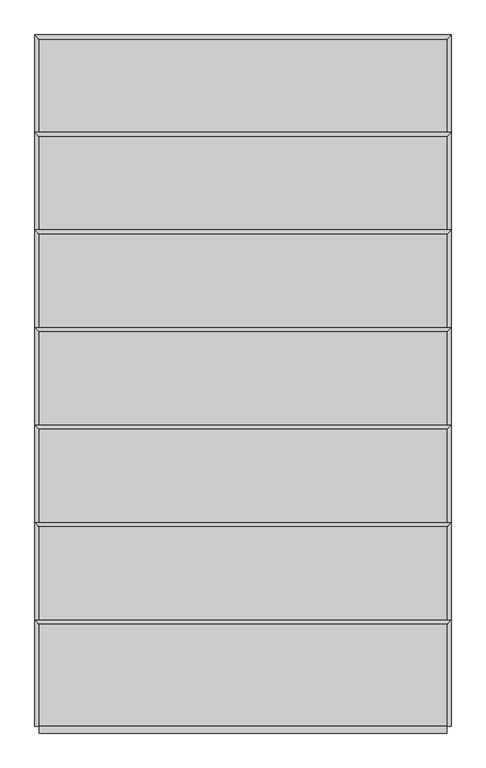
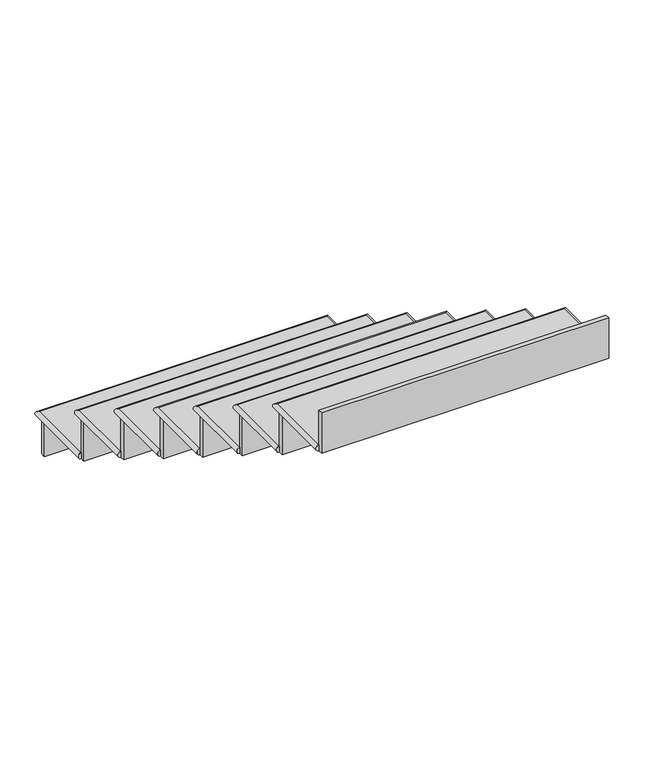
"""IFC4 building model written with IfcOpenShell, lengths in millimetres: stair flight geometry."""

import ifcopenshell
import ifcopenshell.guid

model = None  # the IFC model being written
_history = None  # IfcOwnerHistory: only IFC2X3 demands one
_inside = {}  # id of a spatial element -> (the spatial element, [elements in it])
_under = {}  # id of a project, library or spatial element -> (it, [spatial elements below it])
_declared = {}  # id of a project -> (the project, [libraries it declares])
_typed = {}  # id of a type object -> (the type object, [elements of that type])
_made_of = {}  # id of a material, layer set ... -> (it, [elements and type objects made of it])


def new_model(schema):
    """Start an empty IFC model of exactly this schema.

    Asked for "IFC4X3", IfcOpenShell would pick the latest addendum, in which some entities
    have other attributes; the version numbers below select the first issue.
    IFC2X3 requires an IfcOwnerHistory on every rooted entity: one is made here for all.
    """
    global model, _history
    if schema == "IFC4X3":
        model = ifcopenshell.file(schema_version=(4, 3, 0, 0))
    else:
        model = ifcopenshell.file(schema=schema)
    _inside.clear()
    _under.clear()
    _declared.clear()
    _typed.clear()
    _made_of.clear()
    _history = None
    if model.schema == "IFC2X3":
        org = make("IfcOrganization", Name="unknown")
        user = make(
            "IfcPersonAndOrganization",
            ThePerson=make("IfcPerson", FamilyName="unknown"),
            TheOrganization=org,
        )
        app = make(
            "IfcApplication",
            ApplicationDeveloper=org,
            Version="unknown",
            ApplicationFullName="unknown",
            ApplicationIdentifier="unknown",
        )
        _history = make(
            "IfcOwnerHistory",
            OwningUser=user,
            OwningApplication=app,
            ChangeAction="ADDED",
            CreationDate=0,
        )
    return model


def make(cls, **values):
    """One entity of the class cls with the attributes given. An attribute that is None is left unset."""
    return model.create_entity(
        cls, **{name: value for name, value in values.items() if value is not None}
    )


def rooted(cls, **values):
    """An entity with a GlobalId (a new one), such as an element, a storey or a relation."""
    return make(cls, GlobalId=ifcopenshell.guid.new(), OwnerHistory=_history, **values)


def si_unit(unit_type, name, prefix=None):
    """IfcSIUnit, for example si_unit("LENGTHUNIT", "METRE", prefix="MILLI")."""
    return make("IfcSIUnit", UnitType=unit_type, Prefix=prefix, Name=name)


def assignment(units):
    """IfcUnitAssignment: the units of a project."""
    return None if units is None else make("IfcUnitAssignment", Units=units)


def point(xyz):
    """IfcCartesianPoint."""
    return None if xyz is None else make("IfcCartesianPoint", Coordinates=xyz)


def direction(xyz):
    """IfcDirection."""
    return None if xyz is None else make("IfcDirection", DirectionRatios=xyz)


def frame(location, z_axis=None, x_axis=None):
    """IfcAxis2Placement3D, a coordinate frame: its origin and axes. An axis left out is left unset."""
    return make(
        "IfcAxis2Placement3D",
        Location=point(location),
        Axis=direction(z_axis),
        RefDirection=direction(x_axis),
    )


def origin():
    """The frame at (0, 0, 0) with its axes left unset."""
    return frame((0.0, 0.0, 0.0))


def place(relative_to, where):
    """IfcLocalPlacement: puts the frame where relative to a parent placement (None: the world)."""
    return make(
        "IfcLocalPlacement", PlacementRelTo=relative_to, RelativePlacement=where
    )


def context(
    kind, dimensions, precision=None, world=None, true_north=None, identifier=None
):
    """IfcGeometricRepresentationContext, for example the 3D "Model" context."""
    return make(
        "IfcGeometricRepresentationContext",
        ContextIdentifier=identifier,
        ContextType=kind,
        CoordinateSpaceDimension=dimensions,
        Precision=precision,
        WorldCoordinateSystem=world,
        TrueNorth=true_north,
    )


def project(units=None, contexts=None):
    """IfcProject with its units and contexts."""
    return rooted(
        "IfcProject",
        Name="project",
        RepresentationContexts=contexts,
        UnitsInContext=assignment(units),
    )


def spatial(cls, under=None, at=None, **own):
    """A site, building, storey or space (cls), placed at a placement, below another one or the project."""
    s = rooted(cls, ObjectPlacement=at, **own)
    if under is not None:
        _under.setdefault(under.id(), (under, []))[1].append(s)
    return s


def circle_curve(where, radius):
    """IfcCircle in the frame where."""
    return make("IfcCircle", Position=where, Radius=radius)


def ellipse_curve(where, semi_axis1, semi_axis2):
    """IfcEllipse in the frame where."""
    return make(
        "IfcEllipse", Position=where, SemiAxis1=semi_axis1, SemiAxis2=semi_axis2
    )


def faces_of(points, faces, orient=None, outer=None):
    """IfcFace entities. A face is a list of loops; a loop is a list of indices into points, from 0.

    orient and outer hold one flag for each loop. By default every Orientation is true, the
    first loop of a face is its IfcFaceOuterBound and the others are IfcFaceBound.
    """
    made = []
    for i, loops in enumerate(faces):
        bounds = []
        for j, loop in enumerate(loops):
            is_outer = j == 0 if outer is None else outer[i][j]
            bounds.append(
                make(
                    "IfcFaceOuterBound" if is_outer else "IfcFaceBound",
                    Bound=make("IfcPolyLoop", Polygon=[points[k] for k in loop]),
                    Orientation=True if orient is None else orient[i][j],
                )
            )
        made.append(make("IfcFace", Bounds=bounds))
    return made


def faceted_brep(points, faces, orient=None, outer=None, voids=None):
    """IfcFacetedBrep: a solid bounded by flat faces; with voids (closed shells), ...WithVoids."""
    shared = [point(p) for p in points]
    hull = make("IfcClosedShell", CfsFaces=faces_of(shared, faces, orient, outer))
    if voids is None:
        return make("IfcFacetedBrep", Outer=hull)
    return make(
        "IfcFacetedBrepWithVoids",
        Outer=hull,
        Voids=[
            make(cls, CfsFaces=faces_of(shared, fs, o, b)) for cls, fs, o, b in voids
        ],
    )


def shape(context_of_items, identifier, shape_type, items):
    """IfcShapeRepresentation: the items that make up one representation, for example the "Body"."""
    return make(
        "IfcShapeRepresentation",
        ContextOfItems=context_of_items,
        RepresentationIdentifier=identifier,
        RepresentationType=shape_type,
        Items=items,
    )


def source(mapping_origin, context_of_items, identifier, shape_type, items):
    """IfcRepresentationMap: a shape defined once, which mapped items show again and again."""
    return make(
        "IfcRepresentationMap",
        MappingOrigin=mapping_origin,
        MappedRepresentation=shape(context_of_items, identifier, shape_type, items),
    )


def transform(
    local_origin,
    x_axis=None,
    y_axis=None,
    z_axis=None,
    scale=None,
    scale2=None,
    scale3=None,
    uniform=True,
):
    """IfcCartesianTransformationOperator3D, or its non-uniform kind. x_axis, y_axis, z_axis: its Axis1, 2, 3."""
    if uniform:
        return make(
            "IfcCartesianTransformationOperator3D",
            Axis1=direction(x_axis),
            Axis2=direction(y_axis),
            LocalOrigin=point(local_origin),
            Scale=scale,
            Axis3=direction(z_axis),
        )
    return make(
        "IfcCartesianTransformationOperator3DnonUniform",
        Axis1=direction(x_axis),
        Axis2=direction(y_axis),
        LocalOrigin=point(local_origin),
        Scale=scale,
        Axis3=direction(z_axis),
        Scale2=scale2,
        Scale3=scale3,
    )


def mapped(mapping_source, mapping_target):
    """IfcMappedItem: shows the shape of a source again, moved by a transform."""
    return make(
        "IfcMappedItem", MappingSource=mapping_source, MappingTarget=mapping_target
    )


def made_of(thing, what):
    """Note that an element or type object is made of a material, layer set ...; save() writes the relation."""
    if what is not None:
        _made_of.setdefault(what.id(), (what, []))[1].append(thing)
    return thing


def element(
    cls,
    number,
    at=None,
    inside=None,
    cuts=None,
    type_object=None,
    material=None,
    context=None,
    identifier="Body",
    shape_type=None,
    held_by="IfcProductDefinitionShape",
    body=None,
    shapes=None,
    **own,
):
    """One element of the class cls, such as IfcWall. Its Tag is "e" and its number.

    at: its placement. inside: the storey or other place that contains it. cuts: it is an
    opening in that element (IfcRelVoidsElement). A single representation is given by context,
    identifier, shape_type and body (its items); several are given by shapes. held_by: the class
    of the entity that holds the representations. save() writes the other relations.
    """
    e = rooted(cls, Tag="e%d" % number, ObjectPlacement=at, **own)
    if body is not None:
        shapes = [shape(context, identifier, shape_type, body)]
    if shapes is not None:
        e.Representation = make(held_by, Representations=shapes)
    if inside is not None:
        _inside.setdefault(inside.id(), (inside, []))[1].append(e)
    if cuts is not None:
        rooted(
            "IfcRelVoidsElement", RelatingBuildingElement=cuts, RelatedOpeningElement=e
        )
    if type_object is not None:
        _typed.setdefault(type_object.id(), (type_object, []))[1].append(e)
    return made_of(e, material)


def aggregate(whole, parts):
    """IfcRelAggregates: a whole, such as a stair, and the parts it consists of."""
    return rooted("IfcRelAggregates", RelatingObject=whole, RelatedObjects=parts)


def save(model, path):
    """Write the relations noted so far, then the file.

    IfcRelAggregates (storeys below a building ...), IfcRelContainedInSpatialStructure (elements
    in a storey), IfcRelDefinesByType, IfcRelAssociatesMaterial and IfcRelDeclares: one each for
    every whole, place, type object, material and project.
    """
    for whole, parts in _under.values():
        aggregate(whole, parts)
    for where, things in _inside.values():
        rooted(
            "IfcRelContainedInSpatialStructure",
            RelatedElements=things,
            RelatingStructure=where,
        )
    for kind, things in _typed.values():
        rooted("IfcRelDefinesByType", RelatedObjects=things, RelatingType=kind)
    for what, things in _made_of.values():
        rooted("IfcRelAssociatesMaterial", RelatedObjects=things, RelatingMaterial=what)
    for by, libraries in _declared.values():
        rooted("IfcRelDeclares", RelatingContext=by, RelatedDefinitions=libraries)
    model.write(path)


def plane_surface(at):
    """IfcPlane: the flat surface through the origin of the frame at, square to its z axis."""
    return make("IfcPlane", Position=at)


def cylinder_surface(at, radius):
    """IfcCylindricalSurface: all points at the distance radius from the z axis of the frame at."""
    return make("IfcCylindricalSurface", Position=at, Radius=radius)


def advanced_brep(points, edges, surfaces, faces):
    """IfcAdvancedBrep: a solid bounded by faces that lie on surfaces and meet in shared edges.

    An edge is (start, end): straight between two places in points (the first is 0);
    or (start, end, curve); or (start, end, curve, False) where it runs against its curve.
    A face is (place in surfaces, loops), or (place, loops, False) where it looks against
    its surface's normal. A loop lists edges by number (the first is 1), with a minus sign
    where the edge is run from its end to its start. The first loop is the outer one.
    """
    corners = [point(p) for p in points]
    vertices = [make("IfcVertexPoint", VertexGeometry=c) for c in corners]
    made = []
    for start, end, *more in edges:
        made.append(
            make(
                "IfcEdgeCurve",
                EdgeStart=vertices[start],
                EdgeEnd=vertices[end],
                EdgeGeometry=more[0] if more else make("IfcPolyline", Points=[corners[start], corners[end]]),
                SameSense=more[1] if len(more) > 1 else True,
            )
        )
    hull = []
    for where, loops, *sense in faces:
        bounds = []
        for j, loop in enumerate(loops):
            ring = [make("IfcOrientedEdge", EdgeElement=made[abs(k) - 1], Orientation=k > 0) for k in loop]
            bounds.append(
                make(
                    "IfcFaceOuterBound" if j == 0 else "IfcFaceBound",
                    Bound=make("IfcEdgeLoop", EdgeList=ring),
                    Orientation=True,
                )
            )
        hull.append(make("IfcAdvancedFace", Bounds=bounds, FaceSurface=surfaces[where], SameSense=sense[0] if sense else True))
    return make("IfcAdvancedBrep", Outer=make("IfcClosedShell", CfsFaces=hull))


def stair_flight_dc9404dc(model_context):
    return source(origin(), model_context, "Body", "SolidModel", [
        advanced_brep(
        [(27220.0620052, 5811.3043237, 149.621875), (27220.0620052, 5811.3043237, 175.021875), (28388.4620052, 5811.3043237, 175.021875), (28388.4620052, 5811.3043237, 149.621875), (27220.0620052, 5519.2043237, 175.021875), (28388.4620052, 5519.2043237, 175.021875), (28388.4620052, 5519.2043237, 149.621875), (27220.0620052, 5519.2043237, 149.621875)],
        [
            (0, 1, ellipse_curve(frame((27220.0620052, 5811.3043237, 162.321875), z_axis=(0.7071067811865434, 0.7071067811865517, 0.0), x_axis=(-0.7071067811865517, 0.7071067811865434, 0.0)), 17.9605122, 12.7)),
            (1, 2),
            (2, 3, ellipse_curve(frame((28388.4620052, 5811.3043237, 162.321875), z_axis=(-0.7071067811865517, 0.7071067811865434, 0.0), x_axis=(-0.7071067811865434, -0.7071067811865516, 0.0)), 17.9605122, 12.7)),
            (3, 0),
            (4, 5),
            (5, 2),
            (1, 4),
            (6, 7),
            (7, 0),
            (3, 6),
            (4, 7, circle_curve(frame((27220.0620052, 5519.2043237, 162.321875), z_axis=(0.0, -1.0, 0.0), x_axis=(1.0, 0.0, 0.0)), 12.7)),
            (6, 5, circle_curve(frame((28388.4620052, 5519.2043237, 162.321875), z_axis=(0.0, -1.0, 0.0), x_axis=(-1.0, 0.0, 0.0)), 12.7)),
        ],
        [
            cylinder_surface(frame((27220.0620052, 5811.3043237, 162.321875), z_axis=(-1.0, 0.0, 0.0), x_axis=(0.0, -1.0, 0.0)), 12.7),
            plane_surface(frame((28388.4620052, 5824.0043237, 175.021875), z_axis=(0.0, 0.0, 1.0), x_axis=(0.0, 1.0, 0.0))),
            plane_surface(frame((28388.4620052, 5824.0043237, 149.621875), z_axis=(0.0, 0.0, -1.0), x_axis=(0.0, -1.0, 0.0))),
            plane_surface(frame((27220.0620052, 5519.2043237, 175.021875), z_axis=(0.0, -1.0, 0.0), x_axis=(0.0, 0.0, -1.0))),
            cylinder_surface(frame((27220.0620052, 5519.2043237, 162.321875), z_axis=(0.0, -1.0, 0.0), x_axis=(1.0, 0.0, 0.0)), 12.7),
            cylinder_surface(frame((28388.4620052, 5811.3043237, 162.321875), z_axis=(0.0, 1.0, 0.0), x_axis=(-1.0, 0.0, 0.0)), 12.7),
        ],
        [
            (0, [[1, 2, 3, 4]]),
            (1, [[5, 6, -2, 7]]),
            (2, [[8, 9, -4, 10]]),
            (3, [[-5, 11, -8, 12]]),
            (4, [[-11, -7, -1, -9]]),
            (5, [[-3, -6, -12, -10]]),
        ],
    ),
        faceted_brep([(27220.0620052, 5798.6043237, 149.621875), (27220.0620052, 5798.6043237, 0.0), (27220.0620052, 5779.5543237, 0.0), (27220.0620052, 5779.5543237, 149.621875), (28388.4620052, 5798.6043237, 149.621875), (28388.4620052, 5779.5543237, 149.621875), (28388.4620052, 5779.5543237, 0.0), (28388.4620052, 5798.6043237, 0.0)], [[[0, 1, 2, 3]], [[4, 5, 6, 7]], [[1, 0, 4, 7]], [[2, 1, 7, 6]], [[3, 2, 6, 5]], [[0, 3, 5, 4]]]),
        faceted_brep([(27220.0620052, 5519.2043237, 324.64375), (27220.0620052, 5519.2043237, 149.621875), (27220.0620052, 5500.1543237, 149.621875), (27220.0620052, 5500.1543237, 324.64375), (28388.4620052, 5519.2043237, 324.64375), (28388.4620052, 5500.1543237, 324.64375), (28388.4620052, 5500.1543237, 149.621875), (28388.4620052, 5519.2043237, 149.621875)], [[[0, 1, 2, 3]], [[4, 5, 6, 7]], [[1, 0, 4, 7]], [[2, 1, 7, 6]], [[3, 2, 6, 5]], [[0, 3, 5, 4]]]),
        advanced_brep(
        [(27220.0620052, 5239.8043237, 350.04375), (28388.4620052, 5239.8043237, 350.04375), (28388.4620052, 5531.9043237, 350.04375), (27220.0620052, 5531.9043237, 350.04375), (28388.4620052, 5239.8043237, 324.64375), (27220.0620052, 5239.8043237, 324.64375), (27220.0620052, 5531.9043237, 324.64375), (28388.4620052, 5531.9043237, 324.64375)],
        [
            (0, 1),
            (1, 2),
            (2, 3),
            (3, 0),
            (4, 5),
            (5, 6),
            (6, 7),
            (7, 4),
            (0, 5, circle_curve(frame((27220.0620052, 5239.8043237, 337.34375), z_axis=(0.0, -1.0, 0.0), x_axis=(1.0, 0.0, 0.0)), 12.7)),
            (4, 1, circle_curve(frame((28388.4620052, 5239.8043237, 337.34375), z_axis=(0.0, -1.0, 0.0), x_axis=(-1.0, 0.0, 0.0)), 12.7)),
            (6, 3, ellipse_curve(frame((27220.0620052, 5531.9043237, 337.34375), z_axis=(0.7071067811865378, 0.7071067811865571, 0.0), x_axis=(-0.7071067811865572, 0.7071067811865377, 0.0)), 17.9605122, 12.7)),
            (2, 7, ellipse_curve(frame((28388.4620052, 5531.9043237, 337.34375), z_axis=(-0.7071067811865572, 0.7071067811865378, 0.0), x_axis=(-0.7071067811865378, -0.7071067811865572, 0.0)), 17.9605122, 12.7)),
        ],
        [
            plane_surface(frame((28388.4620052, 5824.0043237, 350.04375), z_axis=(0.0, 0.0, 1.0), x_axis=(0.0, 1.0, 0.0))),
            plane_surface(frame((28388.4620052, 5824.0043237, 324.64375), z_axis=(0.0, 0.0, -1.0), x_axis=(0.0, -1.0, 0.0))),
            plane_surface(frame((27220.0620052, 5239.8043237, 350.04375), z_axis=(0.0, -1.0, 0.0), x_axis=(0.0, 0.0, -1.0))),
            cylinder_surface(frame((27220.0620052, 5531.9043237, 337.34375), z_axis=(-1.0, 0.0, 0.0), x_axis=(0.0, -1.0, 0.0)), 12.7),
            cylinder_surface(frame((27220.0620052, 5239.8043237, 337.34375), z_axis=(0.0, -1.0, 0.0), x_axis=(1.0, 0.0, 0.0)), 12.7),
            cylinder_surface(frame((28388.4620052, 5531.9043237, 337.34375), z_axis=(0.0, 1.0, 0.0), x_axis=(-1.0, 0.0, 0.0)), 12.7),
        ],
        [
            (0, [[1, 2, 3, 4]]),
            (1, [[5, 6, 7, 8]]),
            (2, [[-1, 9, -5, 10]]),
            (3, [[11, -3, 12, -7]]),
            (4, [[-9, -4, -11, -6]]),
            (5, [[-12, -2, -10, -8]]),
        ],
    ),
        faceted_brep([(27220.0620052, 5239.8043237, 499.665625), (27220.0620052, 5239.8043237, 324.64375), (27220.0620052, 5220.7543237, 324.64375), (27220.0620052, 5220.7543237, 499.665625), (28388.4620052, 5239.8043237, 499.665625), (28388.4620052, 5220.7543237, 499.665625), (28388.4620052, 5220.7543237, 324.64375), (28388.4620052, 5239.8043237, 324.64375)], [[[0, 1, 2, 3]], [[4, 5, 6, 7]], [[1, 0, 4, 7]], [[2, 1, 7, 6]], [[3, 2, 6, 5]], [[0, 3, 5, 4]]]),
        advanced_brep(
        [(27220.0620052, 4960.4043237, 525.065625), (28388.4620052, 4960.4043237, 525.065625), (28388.4620052, 5252.5043237, 525.065625), (27220.0620052, 5252.5043237, 525.065625), (28388.4620052, 4960.4043237, 499.665625), (27220.0620052, 4960.4043237, 499.665625), (27220.0620052, 5252.5043237, 499.665625), (28388.4620052, 5252.5043237, 499.665625)],
        [
            (0, 1),
            (1, 2),
            (2, 3),
            (3, 0),
            (4, 5),
            (5, 6),
            (6, 7),
            (7, 4),
            (0, 5, circle_curve(frame((27220.0620052, 4960.4043237, 512.365625), z_axis=(0.0, -1.0, 0.0), x_axis=(1.0, 0.0, 0.0)), 12.7)),
            (4, 1, circle_curve(frame((28388.4620052, 4960.4043237, 512.365625), z_axis=(0.0, -1.0, 0.0), x_axis=(-1.0, 0.0, 0.0)), 12.7)),
            (6, 3, ellipse_curve(frame((27220.0620052, 5252.5043237, 512.365625), z_axis=(0.7071067811865378, 0.7071067811865571, 0.0), x_axis=(-0.7071067811865572, 0.7071067811865377, 0.0)), 17.9605122, 12.7)),
            (2, 7, ellipse_curve(frame((28388.4620052, 5252.5043237, 512.365625), z_axis=(-0.7071067811865572, 0.7071067811865378, 0.0), x_axis=(-0.7071067811865378, -0.7071067811865572, 0.0)), 17.9605122, 12.7)),
        ],
        [
            plane_surface(frame((28388.4620052, 5544.6043237, 525.065625), z_axis=(0.0, 0.0, 1.0), x_axis=(0.0, 1.0, 0.0))),
            plane_surface(frame((28388.4620052, 5544.6043237, 499.665625), z_axis=(0.0, 0.0, -1.0), x_axis=(0.0, -1.0, 0.0))),
            plane_surface(frame((27220.0620052, 4960.4043237, 525.065625), z_axis=(0.0, -1.0, 0.0), x_axis=(0.0, 0.0, -1.0))),
            cylinder_surface(frame((27220.0620052, 5252.5043237, 512.365625), z_axis=(-1.0, 0.0, 0.0), x_axis=(0.0, -1.0, 0.0)), 12.7),
            cylinder_surface(frame((27220.0620052, 4960.4043237, 512.365625), z_axis=(0.0, -1.0, 0.0), x_axis=(1.0, 0.0, 0.0)), 12.7),
            cylinder_surface(frame((28388.4620052, 5252.5043237, 512.365625), z_axis=(0.0, 1.0, 0.0), x_axis=(-1.0, 0.0, 0.0)), 12.7),
        ],
        [
            (0, [[1, 2, 3, 4]]),
            (1, [[5, 6, 7, 8]]),
            (2, [[-1, 9, -5, 10]]),
            (3, [[11, -3, 12, -7]]),
            (4, [[-9, -4, -11, -6]]),
            (5, [[-12, -2, -10, -8]]),
        ],
    ),
        faceted_brep([(27220.0620052, 4960.4043237, 674.6875), (27220.0620052, 4960.4043237, 499.665625), (27220.0620052, 4941.3543237, 499.665625), (27220.0620052, 4941.3543237, 674.6875), (28388.4620052, 4960.4043237, 674.6875), (28388.4620052, 4941.3543237, 674.6875), (28388.4620052, 4941.3543237, 499.665625), (28388.4620052, 4960.4043237, 499.665625)], [[[0, 1, 2, 3]], [[4, 5, 6, 7]], [[1, 0, 4, 7]], [[2, 1, 7, 6]], [[3, 2, 6, 5]], [[0, 3, 5, 4]]]),
        advanced_brep(
        [(27220.0620052, 4681.0043237, 700.0875), (28388.4620052, 4681.0043237, 700.0875), (28388.4620052, 4973.1043237, 700.0875), (27220.0620052, 4973.1043237, 700.0875), (28388.4620052, 4681.0043237, 674.6875), (27220.0620052, 4681.0043237, 674.6875), (27220.0620052, 4973.1043237, 674.6875), (28388.4620052, 4973.1043237, 674.6875)],
        [
            (0, 1),
            (1, 2),
            (2, 3),
            (3, 0),
            (4, 5),
            (5, 6),
            (6, 7),
            (7, 4),
            (0, 5, circle_curve(frame((27220.0620052, 4681.0043237, 687.3875), z_axis=(0.0, -1.0, 0.0), x_axis=(1.0, 0.0, 0.0)), 12.7)),
            (4, 1, circle_curve(frame((28388.4620052, 4681.0043237, 687.3875), z_axis=(0.0, -1.0, 0.0), x_axis=(-1.0, 0.0, 0.0)), 12.7)),
            (6, 3, ellipse_curve(frame((27220.0620052, 4973.1043237, 687.3875), z_axis=(0.7071067811865378, 0.7071067811865571, 0.0), x_axis=(-0.7071067811865572, 0.7071067811865377, 0.0)), 17.9605122, 12.7)),
            (2, 7, ellipse_curve(frame((28388.4620052, 4973.1043237, 687.3875), z_axis=(-0.7071067811865572, 0.7071067811865378, 0.0), x_axis=(-0.7071067811865378, -0.7071067811865572, 0.0)), 17.9605122, 12.7)),
        ],
        [
            plane_surface(frame((28388.4620052, 5265.2043237, 700.0875), z_axis=(0.0, 0.0, 1.0), x_axis=(0.0, 1.0, 0.0))),
            plane_surface(frame((28388.4620052, 5265.2043237, 674.6875), z_axis=(0.0, 0.0, -1.0), x_axis=(0.0, -1.0, 0.0))),
            plane_surface(frame((27220.0620052, 4681.0043237, 700.0875), z_axis=(0.0, -1.0, 0.0), x_axis=(0.0, 0.0, -1.0))),
            cylinder_surface(frame((27220.0620052, 4973.1043237, 687.3875), z_axis=(-1.0, 0.0, 0.0), x_axis=(0.0, -1.0, 0.0)), 12.7),
            cylinder_surface(frame((27220.0620052, 4681.0043237, 687.3875), z_axis=(0.0, -1.0, 0.0), x_axis=(1.0, 0.0, 0.0)), 12.7),
            cylinder_surface(frame((28388.4620052, 4973.1043237, 687.3875), z_axis=(0.0, 1.0, 0.0), x_axis=(-1.0, 0.0, 0.0)), 12.7),
        ],
        [
            (0, [[1, 2, 3, 4]]),
            (1, [[5, 6, 7, 8]]),
            (2, [[-1, 9, -5, 10]]),
            (3, [[11, -3, 12, -7]]),
            (4, [[-9, -4, -11, -6]]),
            (5, [[-12, -2, -10, -8]]),
        ],
    ),
        faceted_brep([(27220.0620052, 4681.0043237, 849.709375), (27220.0620052, 4681.0043237, 674.6875), (27220.0620052, 4661.9543237, 674.6875), (27220.0620052, 4661.9543237, 849.709375), (28388.4620052, 4681.0043237, 849.709375), (28388.4620052, 4661.9543237, 849.709375), (28388.4620052, 4661.9543237, 674.6875), (28388.4620052, 4681.0043237, 674.6875)], [[[0, 1, 2, 3]], [[4, 5, 6, 7]], [[1, 0, 4, 7]], [[2, 1, 7, 6]], [[3, 2, 6, 5]], [[0, 3, 5, 4]]]),
        advanced_brep(
        [(27220.0620052, 4401.6043237, 875.109375), (28388.4620052, 4401.6043237, 875.109375), (28388.4620052, 4693.7043237, 875.109375), (27220.0620052, 4693.7043237, 875.109375), (28388.4620052, 4401.6043237, 849.709375), (27220.0620052, 4401.6043237, 849.709375), (27220.0620052, 4693.7043237, 849.709375), (28388.4620052, 4693.7043237, 849.709375)],
        [
            (0, 1),
            (1, 2),
            (2, 3),
            (3, 0),
            (4, 5),
            (5, 6),
            (6, 7),
            (7, 4),
            (0, 5, circle_curve(frame((27220.0620052, 4401.6043237, 862.409375), z_axis=(0.0, -1.0, 0.0), x_axis=(1.0, 0.0, 0.0)), 12.7)),
            (4, 1, circle_curve(frame((28388.4620052, 4401.6043237, 862.409375), z_axis=(0.0, -1.0, 0.0), x_axis=(-1.0, 0.0, 0.0)), 12.7)),
            (6, 3, ellipse_curve(frame((27220.0620052, 4693.7043237, 862.409375), z_axis=(0.7071067811865378, 0.7071067811865571, 0.0), x_axis=(-0.7071067811865572, 0.7071067811865377, 0.0)), 17.9605122, 12.7)),
            (2, 7, ellipse_curve(frame((28388.4620052, 4693.7043237, 862.409375), z_axis=(-0.7071067811865572, 0.7071067811865378, 0.0), x_axis=(-0.7071067811865378, -0.7071067811865572, 0.0)), 17.9605122, 12.7)),
        ],
        [
            plane_surface(frame((28388.4620052, 4985.8043237, 875.109375), z_axis=(0.0, 0.0, 1.0), x_axis=(0.0, 1.0, 0.0))),
            plane_surface(frame((28388.4620052, 4985.8043237, 849.709375), z_axis=(0.0, 0.0, -1.0), x_axis=(0.0, -1.0, 0.0))),
            plane_surface(frame((27220.0620052, 4401.6043237, 875.109375), z_axis=(0.0, -1.0, 0.0), x_axis=(0.0, 0.0, -1.0))),
            cylinder_surface(frame((27220.0620052, 4693.7043237, 862.409375), z_axis=(-1.0, 0.0, 0.0), x_axis=(0.0, -1.0, 0.0)), 12.7),
            cylinder_surface(frame((27220.0620052, 4401.6043237, 862.409375), z_axis=(0.0, -1.0, 0.0), x_axis=(1.0, 0.0, 0.0)), 12.7),
            cylinder_surface(frame((28388.4620052, 4693.7043237, 862.409375), z_axis=(0.0, 1.0, 0.0), x_axis=(-1.0, 0.0, 0.0)), 12.7),
        ],
        [
            (0, [[1, 2, 3, 4]]),
            (1, [[5, 6, 7, 8]]),
            (2, [[-1, 9, -5, 10]]),
            (3, [[11, -3, 12, -7]]),
            (4, [[-9, -4, -11, -6]]),
            (5, [[-12, -2, -10, -8]]),
        ],
    ),
        faceted_brep([(27220.0620052, 4401.6043237, 1024.73125), (27220.0620052, 4401.6043237, 849.709375), (27220.0620052, 4382.5543237, 849.709375), (27220.0620052, 4382.5543237, 1024.73125), (28388.4620052, 4401.6043237, 1024.73125), (28388.4620052, 4382.5543237, 1024.73125), (28388.4620052, 4382.5543237, 849.709375), (28388.4620052, 4401.6043237, 849.709375)], [[[0, 1, 2, 3]], [[4, 5, 6, 7]], [[1, 0, 4, 7]], [[2, 1, 7, 6]], [[3, 2, 6, 5]], [[0, 3, 5, 4]]]),
        advanced_brep(
        [(27220.0620052, 4122.2043237, 1050.13125), (28388.4620052, 4122.2043237, 1050.13125), (28388.4620052, 4414.3043237, 1050.13125), (27220.0620052, 4414.3043237, 1050.13125), (28388.4620052, 4122.2043237, 1024.73125), (27220.0620052, 4122.2043237, 1024.73125), (27220.0620052, 4414.3043237, 1024.73125), (28388.4620052, 4414.3043237, 1024.73125)],
        [
            (0, 1),
            (1, 2),
            (2, 3),
            (3, 0),
            (4, 5),
            (5, 6),
            (6, 7),
            (7, 4),
            (0, 5, circle_curve(frame((27220.0620052, 4122.2043237, 1037.43125), z_axis=(0.0, -1.0, 0.0), x_axis=(1.0, 0.0, 0.0)), 12.7)),
            (4, 1, circle_curve(frame((28388.4620052, 4122.2043237, 1037.43125), z_axis=(0.0, -1.0, 0.0), x_axis=(-1.0, 0.0, 0.0)), 12.7)),
            (6, 3, ellipse_curve(frame((27220.0620052, 4414.3043237, 1037.43125), z_axis=(0.7071067811865378, 0.7071067811865571, 0.0), x_axis=(-0.7071067811865572, 0.7071067811865377, 0.0)), 17.9605122, 12.7)),
            (2, 7, ellipse_curve(frame((28388.4620052, 4414.3043237, 1037.43125), z_axis=(-0.7071067811865572, 0.7071067811865378, 0.0), x_axis=(-0.7071067811865378, -0.7071067811865572, 0.0)), 17.9605122, 12.7)),
        ],
        [
            plane_surface(frame((28388.4620052, 4706.4043237, 1050.13125), z_axis=(0.0, 0.0, 1.0), x_axis=(0.0, 1.0, 0.0))),
            plane_surface(frame((28388.4620052, 4706.4043237, 1024.73125), z_axis=(0.0, 0.0, -1.0), x_axis=(0.0, -1.0, 0.0))),
            plane_surface(frame((27220.0620052, 4122.2043237, 1050.13125), z_axis=(0.0, -1.0, 0.0), x_axis=(0.0, 0.0, -1.0))),
            cylinder_surface(frame((27220.0620052, 4414.3043237, 1037.43125), z_axis=(-1.0, 0.0, 0.0), x_axis=(0.0, -1.0, 0.0)), 12.7),
            cylinder_surface(frame((27220.0620052, 4122.2043237, 1037.43125), z_axis=(0.0, -1.0, 0.0), x_axis=(1.0, 0.0, 0.0)), 12.7),
            cylinder_surface(frame((28388.4620052, 4414.3043237, 1037.43125), z_axis=(0.0, 1.0, 0.0), x_axis=(-1.0, 0.0, 0.0)), 12.7),
        ],
        [
            (0, [[1, 2, 3, 4]]),
            (1, [[5, 6, 7, 8]]),
            (2, [[-1, 9, -5, 10]]),
            (3, [[11, -3, 12, -7]]),
            (4, [[-9, -4, -11, -6]]),
            (5, [[-12, -2, -10, -8]]),
        ],
    ),
        faceted_brep([(27220.0620052, 4122.2043237, 1199.753125), (27220.0620052, 4122.2043237, 1024.73125), (27220.0620052, 4103.1543237, 1024.73125), (27220.0620052, 4103.1543237, 1199.753125), (28388.4620052, 4122.2043237, 1199.753125), (28388.4620052, 4103.1543237, 1199.753125), (28388.4620052, 4103.1543237, 1024.73125), (28388.4620052, 4122.2043237, 1024.73125)], [[[0, 1, 2, 3]], [[4, 5, 6, 7]], [[1, 0, 4, 7]], [[2, 1, 7, 6]], [[3, 2, 6, 5]], [[0, 3, 5, 4]]]),
        faceted_brep([(27220.0620052, 3842.8043237, 1374.775), (27220.0620052, 3842.8043237, 1199.753125), (27220.0620052, 3823.7543237, 1199.753125), (27220.0620052, 3823.7543237, 1374.775), (28388.4620052, 3842.8043237, 1374.775), (28388.4620052, 3823.7543237, 1374.775), (28388.4620052, 3823.7543237, 1199.753125), (28388.4620052, 3842.8043237, 1199.753125)], [[[0, 1, 2, 3]], [[4, 5, 6, 7]], [[1, 0, 4, 7]], [[2, 1, 7, 6]], [[3, 2, 6, 5]], [[0, 3, 5, 4]]]),
        advanced_brep(
        [(27220.0620052, 3842.8043237, 1225.153125), (28388.4620052, 3842.8043237, 1225.153125), (28388.4620052, 4134.9043237, 1225.153125), (27220.0620052, 4134.9043237, 1225.153125), (28388.4620052, 3842.8043237, 1199.753125), (27220.0620052, 3842.8043237, 1199.753125), (27220.0620052, 4134.9043237, 1199.753125), (28388.4620052, 4134.9043237, 1199.753125)],
        [
            (0, 1),
            (1, 2),
            (2, 3),
            (3, 0),
            (4, 5),
            (5, 6),
            (6, 7),
            (7, 4),
            (0, 5, circle_curve(frame((27220.0620052, 3842.8043237, 1212.453125), z_axis=(0.0, -1.0, 0.0), x_axis=(1.0, 0.0, 0.0)), 12.7)),
            (4, 1, circle_curve(frame((28388.4620052, 3842.8043237, 1212.453125), z_axis=(0.0, -1.0, 0.0), x_axis=(-1.0, 0.0, 0.0)), 12.7)),
            (6, 3, ellipse_curve(frame((27220.0620052, 4134.9043237, 1212.453125), z_axis=(0.707106781186535, 0.70710678118656, 0.0), x_axis=(-0.70710678118656, 0.707106781186535, 0.0)), 17.9605122, 12.7)),
            (2, 7, ellipse_curve(frame((28388.4620052, 4134.9043237, 1212.453125), z_axis=(-0.7071067811865601, 0.707106781186535, 0.0), x_axis=(-0.7071067811865349, -0.70710678118656, 0.0)), 17.9605122, 12.7)),
        ],
        [
            plane_surface(frame((28388.4620052, 4427.0043237, 1225.153125), z_axis=(0.0, 0.0, 1.0), x_axis=(0.0, 1.0, 0.0))),
            plane_surface(frame((28388.4620052, 4427.0043237, 1199.753125), z_axis=(0.0, 0.0, -1.0), x_axis=(0.0, -1.0, 0.0))),
            plane_surface(frame((27220.0620052, 3842.8043237, 1225.153125), z_axis=(0.0, -1.0, 0.0), x_axis=(0.0, 0.0, -1.0))),
            cylinder_surface(frame((27220.0620052, 4134.9043237, 1212.453125), z_axis=(-1.0, 0.0, 0.0), x_axis=(0.0, -1.0, 0.0)), 12.7),
            cylinder_surface(frame((27220.0620052, 3842.8043237, 1212.453125), z_axis=(0.0, -1.0, 0.0), x_axis=(1.0, 0.0, 0.0)), 12.7),
            cylinder_surface(frame((28388.4620052, 4134.9043237, 1212.453125), z_axis=(0.0, 1.0, 0.0), x_axis=(-1.0, 0.0, 0.0)), 12.7),
        ],
        [
            (0, [[1, 2, 3, 4]]),
            (1, [[5, 6, 7, 8]]),
            (2, [[-1, 9, -5, 10]]),
            (3, [[11, -3, 12, -7]]),
            (4, [[-9, -4, -11, -6]]),
            (5, [[-12, -2, -10, -8]]),
        ],
    ),
    ])


if __name__ == "__main__":
    model = new_model("IFC4")
    model_context = context("Model", 3, world=origin())
    ifc_project = project(units=[si_unit("LENGTHUNIT", "METRE", prefix="MILLI")], contexts=[model_context])
    site = spatial("IfcSite", under=ifc_project)
    building = spatial("IfcBuilding", under=site)
    placement = place(None, origin())
    stair_flight_shape = stair_flight_dc9404dc(model_context)
    element("IfcStairFlight", 1, at=placement, inside=building, context=model_context, shape_type="MappedRepresentation", body=[
        mapped(stair_flight_shape, transform((0.0, 0.0, 0.0), x_axis=(1.0, 0.0, 0.0), y_axis=(0.0, 1.0, 0.0), z_axis=(0.0, 0.0, 1.0))),
    ])
    save(model, "model.ifc")

# Revit data of these elements
# Element 1 (IfcStairFlight)
#   Materials on its faces: "FINISH T.B.D."
# Materials
#   "FINISH T.B.D.": class "Generic", colour RGB 227 188 136, transparency 0, Cost = 0
